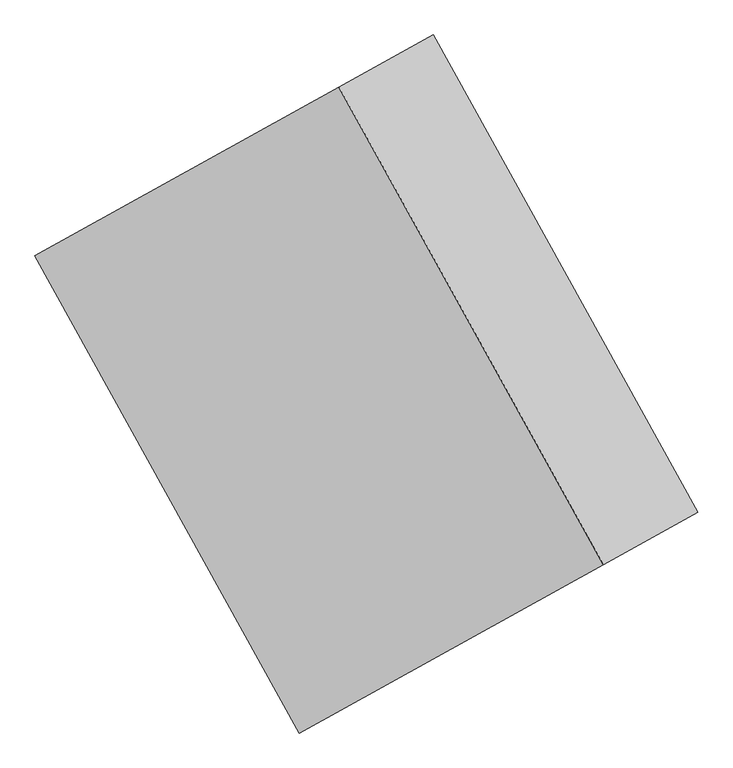
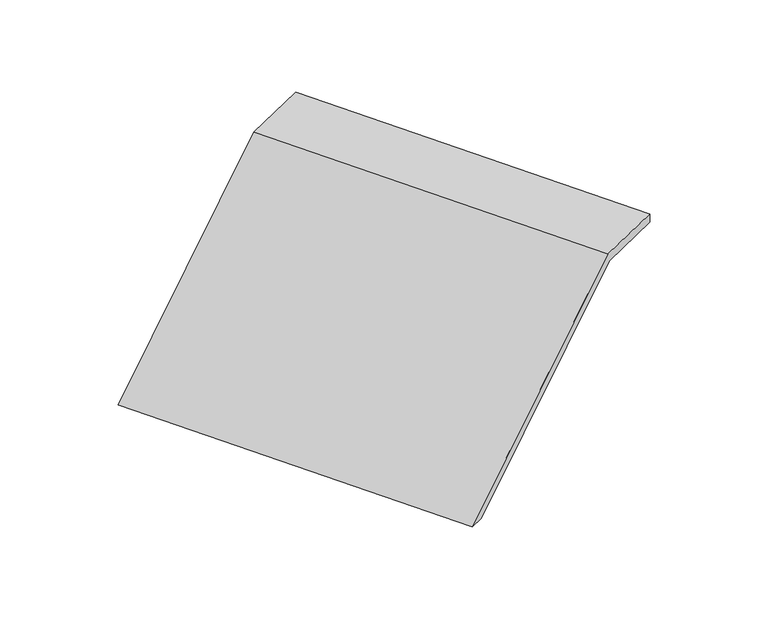
"""IFC4 building model written with IfcOpenShell, lengths in millimetres: beam geometry, KNA_Sf_Talud 4 : KNA_Sf_Talud 4."""

from ifc_helpers import new_model, si_unit, frame, origin, place, context, project, spatial, polyline, outline, extrude, source, transform, mapped, element, save


def beam_7e0037b7(model_context):
    return source(origin(), model_context, "Body", "SweptSolid", [
        extrude(outline(polyline([(2514.9793546, 0.0), (10600.0, -5390.0), (10059.1663525, -5390.0), (2424.1468564, -300.0), (0.0, -300.0), (0.0, 0.0), (2514.9793546, 0.0)])), frame((171930.9778737, -31408.4563133, 4350.0), z_axis=(-0.48434294505380965, 0.874878226713068, 0.0), x_axis=(-0.874878226713068, -0.48434294505380965, 0.0)), (0.0, 0.0, 1.0), 12698.4872578),
    ])


if __name__ == "__main__":
    model = new_model("IFC4")
    model_context = context("Model", 3, world=origin())
    ifc_project = project(units=[si_unit("LENGTHUNIT", "METRE", prefix="MILLI")], contexts=[model_context])
    site = spatial("IfcSite", under=ifc_project)
    building = spatial("IfcBuilding", under=site)
    placement = place(None, origin())
    beam_shape = beam_7e0037b7(model_context)
    element("IfcBeam", 1, ObjectType="KNA_Sf_Talud 4 : KNA_Sf_Talud 4", at=placement, inside=building, context=model_context, shape_type="MappedRepresentation", body=[
        mapped(beam_shape, transform((0.0, 0.0, 0.0), x_axis=(1.0, 0.0, 0.0), y_axis=(0.0, 1.0, 0.0), z_axis=(0.0, 0.0, 1.0))),
    ])
    save(model, "model.ifc")
